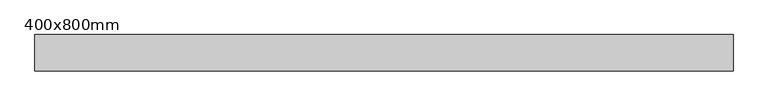
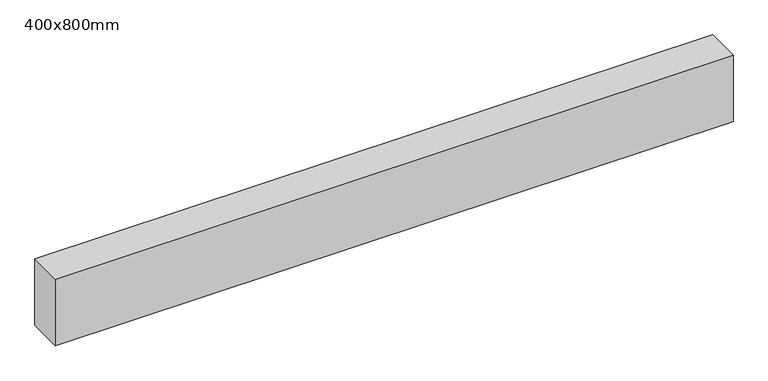
"""IFC4 building model written with IfcOpenShell, lengths in millimetres: beam geometry, S-Frame_CastInPlace_Rectangular : 400x800mm."""

from ifc_helpers import new_model, si_unit, frame, origin, place, context, project, spatial, polyline, outline, extrude, source, transform, mapped, element, save


def beam_400x800mm_1e0f6873(model_context):
    return source(origin(), model_context, "Body", "SweptSolid", [
        extrude(outline(polyline([(3850.0, 200.0), (3850.0, -200.0), (-3850.0, -200.0), (-3850.0, 200.0), (3850.0, 200.0)])), frame((0.0, 0.0, -400.0), z_axis=(0.0, 0.0, 1.0), x_axis=(1.0, 0.0, 0.0)), (0.0, 0.0, 1.0), 800.0),
    ])


if __name__ == "__main__":
    model = new_model("IFC4")
    model_context = context("Model", 3, world=origin())
    ifc_project = project(units=[si_unit("LENGTHUNIT", "METRE", prefix="MILLI")], contexts=[model_context])
    site = spatial("IfcSite", under=ifc_project)
    building = spatial("IfcBuilding", under=site)
    placement = place(None, origin())
    beam_400x800mm_shape = beam_400x800mm_1e0f6873(model_context)
    element("IfcBeam", 1, ObjectType="S-Frame_CastInPlace_Rectangular : 400x800mm", at=placement, inside=building, context=model_context, shape_type="MappedRepresentation", body=[
        mapped(beam_400x800mm_shape, transform((0.0, 0.0, 0.0), x_axis=(1.0, 0.0, 0.0), y_axis=(0.0, 1.0, 0.0), z_axis=(0.0, 0.0, 1.0))),
    ])
    save(model, "model.ifc")

# Revit data of these elements
# Type "S-Frame_CastInPlace_Rectangular : 400x800mm"
#   NS3457-8 Code = "ABA"
#   NS3451 Code = "2230"
#   NS3457-8 = "ABA Konstruktive bjelker"
#   NS3451 = "2230 Bjelker"
#   ModelBy = "Norconsult AS"
#   Manufacturer = "Norconsult"
#   Width = 400 mm
#   Height = 800 mm
#   Length [instance default] = 1524 mm
#   Structural Material = NO_Betong - Plasstøpt
#   Assembly Code = ""
# Element 1 (IfcBeam, "S-Frame_CastInPlace_Rectangular : 400x800mm")
#   Materials on its faces: "NO_Betong - Plasstøpt"
# Materials
#   "NO_Betong - Plasstøpt": class "Betong", colour RGB 186 186 186, transparency 0, Material PI-Name = "Betong B45. 120 kg armering pr m3 betong. Lavkarbonklasse B", Cost = 0, Material CO2e = 230.00 kg/m³
